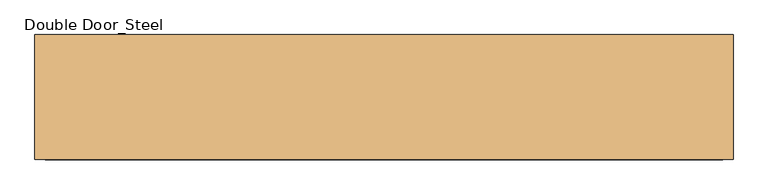
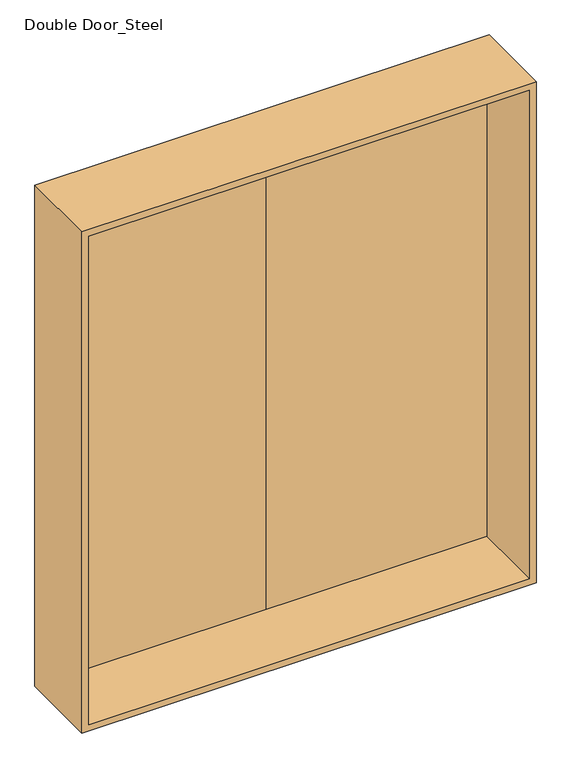
"""IFC4 building model written with IfcOpenShell, lengths in millimetres: door geometry, Double Door_Steel : H_DR_AMB_Double Door_Steel_W2400xH2800."""

from ifc_helpers import new_model, si_unit, frame, origin, place, context, project, spatial, polyline, outline, extrude, faceted_brep, source, transform, mapped, element, save


def double_door_steel_f76c4a76(model_context):
    return source(origin(), model_context, "Body", "SolidModel", [
        extrude(outline(polyline([(1180.0, 175.0), (0.0, 175.0), (0.0, 215.0), (1180.0, 215.0), (1180.0, 175.0)])), frame((0.0, 0.0, 20.0), z_axis=(0.0, 0.0, 1.0), x_axis=(1.0, 0.0, 0.0)), (0.0, 0.0, 1.0), 2760.0),
        extrude(outline(polyline([(0.0, 175.0), (-1180.0, 175.0), (-1180.0, 215.0), (0.0, 215.0), (0.0, 175.0)])), frame((0.0, 0.0, 20.0), z_axis=(0.0, 0.0, 1.0), x_axis=(1.0, 0.0, 0.0)), (0.0, 0.0, 1.0), 2760.0),
        faceted_brep([(1200.0, -215.0, 0.0), (1200.0, 215.0, 0.0), (1200.0, 215.0, 2800.0), (1200.0, -215.0, 2800.0), (-1200.0, 215.0, 2800.0), (-1200.0, -215.0, 2800.0), (-1200.0, 215.0, 0.0), (1180.0, 215.0, 2780.0), (-1180.0, 215.0, 2780.0), (-1180.0, 215.0, 20.0), (1180.0, 215.0, 20.0), (-1200.0, -215.0, 0.0), (1165.0, -215.0, 35.0), (-1165.0, -215.0, 35.0), (-1165.0, -215.0, 2765.0), (1165.0, -215.0, 2765.0), (1165.0, 175.0, 35.0), (1165.0, 175.0, 2765.0), (-1165.0, 175.0, 2765.0), (-1165.0, 175.0, 35.0), (1180.0, 175.0, 20.0), (-1180.0, 175.0, 20.0), (-1180.0, 175.0, 2780.0), (1180.0, 175.0, 2780.0)], [[[0, 1, 2, 3]], [[3, 2, 4, 5]], [[1, 6, 4, 2], [7, 8, 9, 10]], [[5, 4, 6, 11]], [[3, 5, 11, 0], [12, 13, 14, 15]], [[16, 12, 15, 17]], [[17, 15, 14, 18]], [[18, 14, 13, 19]], [[20, 21, 22, 23], [17, 18, 19, 16]], [[10, 20, 23, 7]], [[7, 23, 22, 8]], [[8, 22, 21, 9]], [[11, 6, 1, 0]], [[19, 13, 12, 16]], [[9, 21, 20, 10]]]),
    ])


if __name__ == "__main__":
    model = new_model("IFC4")
    model_context = context("Model", 3, world=origin())
    ifc_project = project(units=[si_unit("LENGTHUNIT", "METRE", prefix="MILLI")], contexts=[model_context])
    site = spatial("IfcSite", under=ifc_project)
    building = spatial("IfcBuilding", under=site)
    placement = place(None, origin())
    double_door_steel_shape = double_door_steel_f76c4a76(model_context)
    element("IfcDoor", 1, ObjectType="Double Door_Steel : H_DR_AMB_Double Door_Steel_W2400xH2800", at=placement, inside=building, context=model_context, shape_type="MappedRepresentation", body=[
        mapped(double_door_steel_shape, transform((0.0, 0.0, 0.0), x_axis=(1.0, 0.0, 0.0), y_axis=(0.0, 1.0, 0.0), z_axis=(0.0, 0.0, 1.0))),
    ])
    save(model, "model.ifc")

# Revit data of these elements
# Type "Double Door_Steel : H_DR_AMB_Double Door_Steel_W2400xH2800"
#   Type Mark = "365"
#   프레임 = ""
#   철물 = ""
#   유리/마감 = ""
#   위치/개소 = ""
#   부호 = "1/SD"
#   문번호 = ""
#   문기호 = "SD"
#   Analytic Construction = "<None>"
#   Height = 2800.000 mm
#   Width = 2400.000 mm
#   Define Thermal Properties by = 1
#   문 틀 = none
#   문 = none
#   Function = (empty or 0)
#   Assembly Code = ""
#   Wall Closure = (empty or 0)
